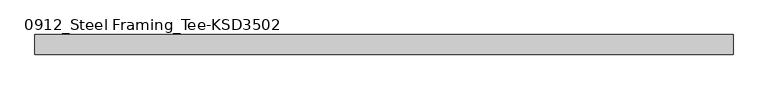
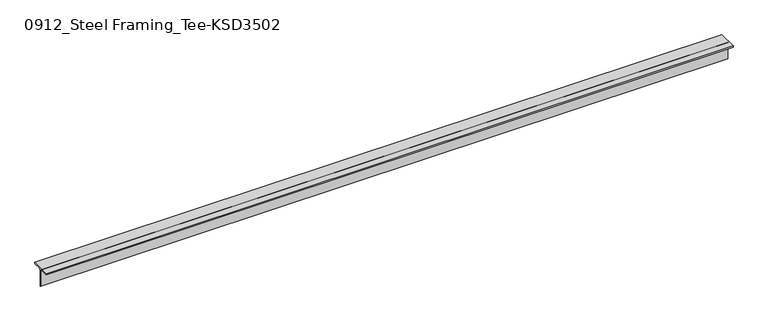
"""IFC4 building model written with IfcOpenShell, lengths in millimetres: member geometry, 0912_Steel Framing_Tee-KSD3502 : H_SB_ASB_CT-150x150x6.5x9."""

from ifc_helpers import new_model, si_unit, point, frame, frame_2d, origin, place, context, project, spatial, polyline, circle_curve, trimmed, segment, composite_curve, outline, extrude, source, transform, mapped, element, save


def member_0912_steel_framing_tee_ksd3502_e3ce81ac(model_context):
    return source(origin(), model_context, "Body", "SweptSolid", [
        extrude(outline(composite_curve([segment(polyline([(-75.0, 75.0), (75.0, 75.0), (75.0, 66.0), (16.25, 66.0)]), True, "CONTINUOUS"), segment(trimmed(circle_curve(frame_2d((16.25, 53.0)), 13.0), [point((16.25, 66.0))], [point((3.25, 53.0))], True, "CARTESIAN"), True, "CONTINUOUS"), segment(polyline([(3.25, 53.0), (3.25, -75.0), (-3.25, -75.0), (-3.25, 53.0)]), True, "CONTINUOUS"), segment(trimmed(circle_curve(frame_2d((-16.25, 53.0)), 13.0), [point((-3.25, 53.0))], [point((-16.25, 66.0))], True, "CARTESIAN"), True, "CONTINUOUS"), segment(polyline([(-16.25, 66.0), (-75.0, 66.0), (-75.0, 75.0)]), True, "CONTINUOUS")], self_intersect=False)), frame((-2577.3, 0.0, 0.0), z_axis=(1.0, 0.0, 0.0), x_axis=(0.0, 1.0, 0.0)), (0.0, 0.0, 1.0), 5329.7),
    ])


if __name__ == "__main__":
    model = new_model("IFC4")
    model_context = context("Model", 3, world=origin())
    ifc_project = project(units=[si_unit("LENGTHUNIT", "METRE", prefix="MILLI")], contexts=[model_context])
    site = spatial("IfcSite", under=ifc_project)
    building = spatial("IfcBuilding", under=site)
    placement = place(None, origin())
    member_0912_steel_framing_tee_ksd3502_shape = member_0912_steel_framing_tee_ksd3502_e3ce81ac(model_context)
    element("IfcMember", 1, ObjectType="0912_Steel Framing_Tee-KSD3502 : H_SB_ASB_CT-150x150x6.5x9", at=placement, inside=building, context=model_context, shape_type="MappedRepresentation", body=[
        mapped(member_0912_steel_framing_tee_ksd3502_shape, transform((0.0, 0.0, 0.0), x_axis=(1.0, 0.0, 0.0), y_axis=(0.0, 1.0, 0.0), z_axis=(0.0, 0.0, 1.0))),
    ])
    save(model, "model.ifc")

# Revit data of these elements
# Type "0912_Steel Framing_Tee-KSD3502 : H_SB_ASB_CT-150x150x6.5x9"
#   H_WM Code_1 = "S01AA003-00001 | Main Steel Structure Fabrication Work | Shelter/Building | Light Steel - Standard (30KG/M>Weight) | Material: (   )"
#   H_WM Code_2 = "S03AA029-00001 | Main Steel Structure Erection Work | Shelter/Building | Light Steel (30KG/M>Weight) | Material: (   )"
#   H_WM Code_3 = "S01AA010-00001 | Main Steel Structure Fabrication Work | Shelter/Building | Steel Painting/Coating | for Non-Fireproofed Steel Surface, Surface Preparation, Primer, Second & Final Coat | Material: (   )"
#   H_Q'ty Cal Type Tag = "SB-Q2"
#   Width = 15.0 cm
#   Web Thickness = 0.65 cm
#   Web Fillet = 1.3 cm
#   Section Area = 23.39 cm²
#   Perimeter = 0.60 m²/m
#   Nominal Weight = 18.40 kgf/m
#   Height = 15.0 cm
#   Flange Thickness = 0.9 cm
#   Centroid Vertical = 7.5 cm
#   Centroid Horizontal = 7.5 cm
#   Length [instance default] = 1.5000 m
#   Structural Material [instance default] = Steel, 45-345
#   Warping Constant = (empty or 0)
#   Torsional Moment of Inertia = 0
#   Section Name Key = ""
#   Plastic Modulus weak axis = 0
#   Plastic Modulus strong axis = 0
#   Moment of Inertia weak axis = 0
#   Moment of Inertia strong axis = 0
#   Elastic Modulus weak axis = 0
#   Elastic Modulus strong axis = 0
#   Bolt Spacing = 0
#   Assembly Code = ""
# Element 1 (IfcMember, "0912_Steel Framing_Tee-KSD3502 : H_SB_ASB_CT-150x150x6.5x9")
#   Structural Material = none
# Materials
#   "Steel, 45-345": class "Metal", colour RGB 189 187 185, transparency 0, Description = "Steel 345 MPa", Cost = 0
